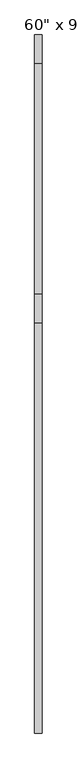
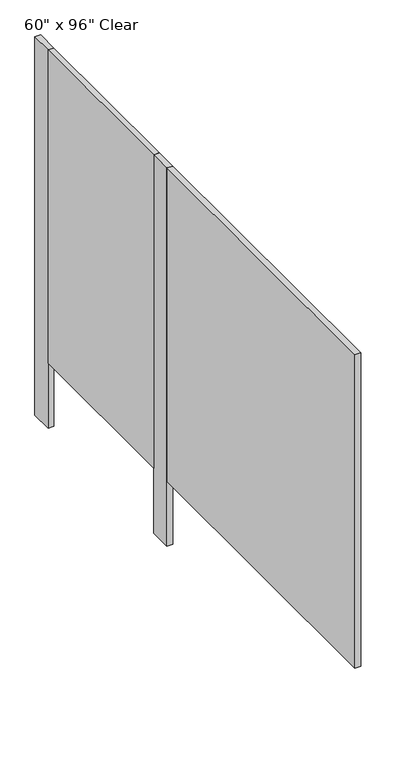
"""IFC4 building model written with IfcOpenShell, lengths in millimetres: proxy geometry."""

from ifc_helpers import new_model, si_unit, frame, origin, origin_with_axes, place, context, project, spatial, polyline, outline, extrude, source, transform, mapped, element, save


def proxy_d530cf2d(model_context):
    return source(origin(), model_context, "Body", "SweptSolid", [
        extrude(outline(polyline([(-661.8968462, 2560.6375), (-661.8968462, 1747.8375), (-687.2968462, 1747.8375), (-687.2968462, 2560.6375), (-661.8968462, 2560.6375)])), frame((0.0, 0.0, 304.8), z_axis=(0.0, 0.0, 1.0), x_axis=(1.0, 0.0, 0.0)), (0.0, 0.0, 1.0), 1473.2),
        extrude(outline(polyline([(-661.8968462, 2662.2375), (-661.8968462, 2560.6375), (-687.2968462, 2560.6375), (-687.2968462, 2662.2375), (-661.8968462, 2662.2375)])), origin_with_axes(), (0.0, 0.0, 1.0), 1778.0),
        extrude(outline(polyline([(-661.8968462, 1747.8375), (-661.8968462, 1646.2375), (-687.2968462, 1646.2375), (-687.2968462, 1747.8375), (-661.8968462, 1747.8375)])), origin_with_axes(), (0.0, 0.0, 1.0), 1778.0),
        extrude(outline(polyline([(-687.2968462, 1646.2375), (-661.8968462, 1646.2375), (-661.8968462, 198.4375), (-687.2968462, 198.4375), (-687.2968462, 1646.2375)])), frame((0.0, 0.0, 304.8), z_axis=(0.0, 0.0, 1.0), x_axis=(1.0, 0.0, 0.0)), (0.0, 0.0, 1.0), 1473.2),
    ])


if __name__ == "__main__":
    model = new_model("IFC4")
    model_context = context("Model", 3, world=origin())
    ifc_project = project(units=[si_unit("LENGTHUNIT", "METRE", prefix="MILLI")], contexts=[model_context])
    site = spatial("IfcSite", under=ifc_project)
    building = spatial("IfcBuilding", under=site)
    placement = place(None, origin())
    proxy_shape = proxy_d530cf2d(model_context)
    element("IfcBuildingElementProxy", 1, Name="Toilet Stall-Accessible-Side-3D w Toilet : 60\" x 96\" Clear", ObjectType="Toilet Stall-Accessible-Side-3D w Toilet : 60\" x 96\" Clear", at=placement, inside=building, context=model_context, shape_type="MappedRepresentation", body=[
        mapped(proxy_shape, transform((0.0, 0.0, 0.0), x_axis=(1.0, 0.0, 0.0), y_axis=(0.0, 1.0, 0.0), z_axis=(0.0, 0.0, 1.0))),
    ])
    save(model, "model.ifc")

# Revit data of these elements
# Type "Toilet Stall-Accessible-Side-3D w Toilet : 60\" x 96\" Clear"
#   Assembly Code = "C1030100"
#   Door Width = 2' - 8"
#   Length = 8' - 0"
#   Width = 5' - 0"
#   Show End Panel [instance default] = yes
#   Toilet Partition Material = Toilet Partition
#   Default Elevation = 0
# Element 1 (IfcBuildingElementProxy, "Toilet Stall-Accessible-Side-3D w Toilet : 60\" x 96\" Clear")
#   Show End Panel = no
#   Materials on its faces: "Toilet Partition"
# Materials
#   "Toilet Partition": class "Unassigned", colour RGB 0 181 188, transparency 0
